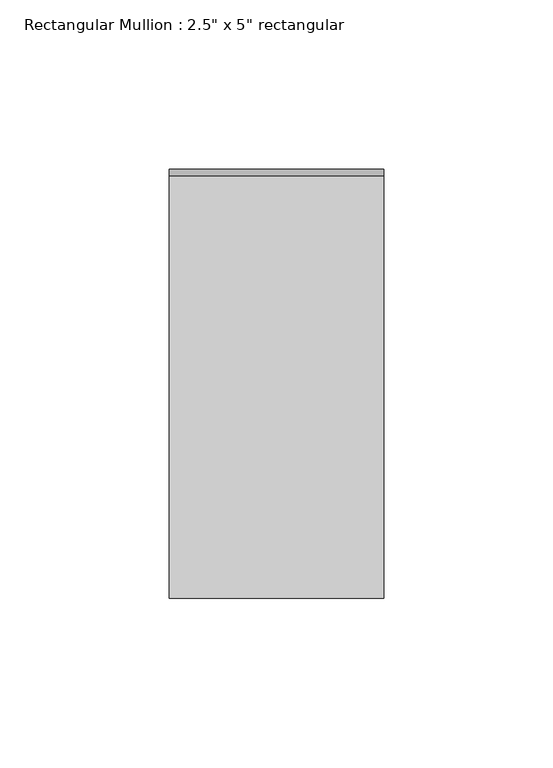
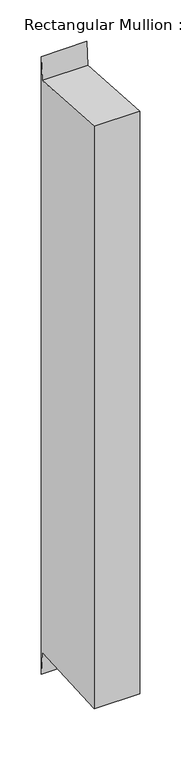
"""IFC4 building model written with IfcOpenShell, lengths in millimetres: member geometry."""

from ifc_helpers import new_model, si_unit, frame, origin, place, context, project, spatial, polyline, outline, extrude, source, transform, mapped, element, save


def member_a397ac22(model_context):
    return source(origin(), model_context, "Body", "SweptSolid", [
        extrude(outline(polyline([(-63.5, 3.8736342), (61.4149606, -3.8662198), (63.5, 29.7846233), (63.5, -880.6846233), (61.4149606, -847.0337802), (-63.5, -854.7736342), (-63.5, 3.8736342)])), frame((-63.5, 0.0, 0.0), z_axis=(1.0, 0.0, 0.0), x_axis=(0.0, 1.0, 0.0)), (0.0, 0.0, 1.0), 63.5),
    ])


if __name__ == "__main__":
    model = new_model("IFC4")
    model_context = context("Model", 3, world=origin())
    ifc_project = project(units=[si_unit("LENGTHUNIT", "METRE", prefix="MILLI")], contexts=[model_context])
    site = spatial("IfcSite", under=ifc_project)
    building = spatial("IfcBuilding", under=site)
    placement = place(None, origin())
    member_shape = member_a397ac22(model_context)
    element("IfcMember", 1, ObjectType="Rectangular Mullion : 2.5\" x 5\" rectangular", at=placement, inside=building, context=model_context, shape_type="MappedRepresentation", body=[
        mapped(member_shape, transform((0.0, 0.0, 0.0), x_axis=(1.0, 0.0, 0.0), y_axis=(0.0, 1.0, 0.0), z_axis=(0.0, 0.0, 1.0))),
    ])
    save(model, "model.ifc")

# Revit data of these elements
# Type "Rectangular Mullion : 2.5\" x 5\" rectangular"
#   built-in parameter 1007304 = 0.416667 (stored number, unit not read)
#   built-in parameter 1007301 = 0.104167 (stored number, unit not read)
#   built-in parameter 1007300 = 0.104167 (stored number, unit not read)
# Element 1 (IfcMember, "Rectangular Mullion : 2.5\" x 5\" rectangular")
#   Materials on its faces: "Metal - Aluminum"
# Materials
#   "Metal - Aluminum": class "Metal", colour RGB 247 247 247, transparency 0, Cost = 0
